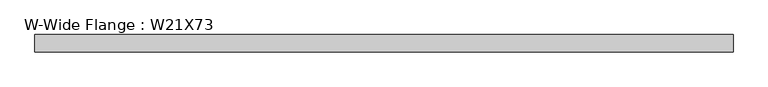
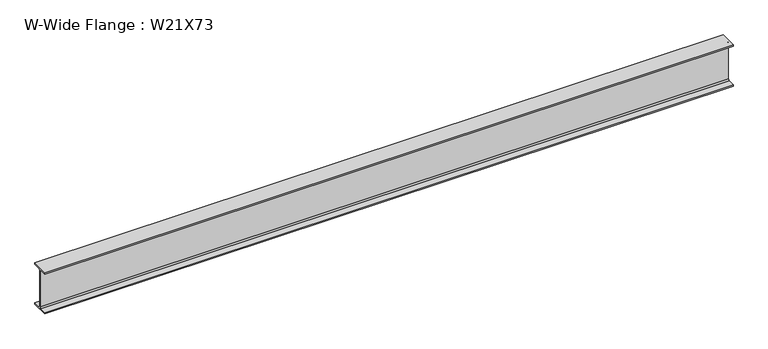
"""IFC4 building model written with IfcOpenShell, lengths in millimetres: beam geometry, W-Wide Flange : W21X73."""

from ifc_helpers import new_model, si_unit, point, frame, frame_2d, origin, place, context, project, spatial, polyline, circle_curve, trimmed, segment, composite_curve, outline, extrude, source, transform, mapped, element, save


def w_wide_flange_w21x73_6fdf119d(model_context):
    return source(origin(), model_context, "Body", "SweptSolid", [
        extrude(outline(composite_curve([segment(polyline([(105.41, -250.444), (105.41, -269.24), (-105.41, -269.24), (-105.41, -250.444), (-23.495, -250.444)]), True, "CONTINUOUS"), segment(trimmed(circle_curve(frame_2d((-23.495, -232.7275)), 17.7165), [point((-23.495, -250.444))], [point((-5.7785, -232.7275))], True, "CARTESIAN"), True, "CONTINUOUS"), segment(polyline([(-5.7785, -232.7275), (-5.7785, 232.7275)]), True, "CONTINUOUS"), segment(trimmed(circle_curve(frame_2d((-23.495, 232.7275)), 17.7165), [point((-5.7785, 232.7275))], [point((-23.495, 250.444))], True, "CARTESIAN"), True, "CONTINUOUS"), segment(polyline([(-23.495, 250.444), (-105.41, 250.444), (-105.41, 269.24), (105.41, 269.24), (105.41, 250.444), (23.495, 250.444)]), True, "CONTINUOUS"), segment(trimmed(circle_curve(frame_2d((23.495, 232.7275)), 17.7165), [point((23.495, 250.444))], [point((5.7785, 232.7275))], True, "CARTESIAN"), True, "CONTINUOUS"), segment(polyline([(5.7785, 232.7275), (5.7785, -232.7275)]), True, "CONTINUOUS"), segment(trimmed(circle_curve(frame_2d((23.495, -232.7275)), 17.7165), [point((5.7785, -232.7275))], [point((23.495, -250.444))], True, "CARTESIAN"), True, "CONTINUOUS"), segment(polyline([(23.495, -250.444), (105.41, -250.444)]), True, "CONTINUOUS")], self_intersect=False)), frame((-4243.07, 0.0, 0.0), z_axis=(1.0, 0.0, 0.0), x_axis=(0.0, 1.0, 0.0)), (0.0, 0.0, 1.0), 8483.6),
    ])


if __name__ == "__main__":
    model = new_model("IFC4")
    model_context = context("Model", 3, world=origin())
    ifc_project = project(units=[si_unit("LENGTHUNIT", "METRE", prefix="MILLI")], contexts=[model_context])
    site = spatial("IfcSite", under=ifc_project)
    building = spatial("IfcBuilding", under=site)
    placement = place(None, origin())
    w_wide_flange_w21x73_shape = w_wide_flange_w21x73_6fdf119d(model_context)
    element("IfcBeam", 1, ObjectType="W-Wide Flange : W21X73", at=placement, inside=building, context=model_context, shape_type="MappedRepresentation", body=[
        mapped(w_wide_flange_w21x73_shape, transform((0.0, 0.0, 0.0), x_axis=(1.0, 0.0, 0.0), y_axis=(0.0, 1.0, 0.0), z_axis=(0.0, 0.0, 1.0))),
    ])
    save(model, "model.ifc")

# Revit data of these elements
# Type "W-Wide Flange : W21X73"
#   Assembly Code = "B10"
#   W = 73
#   Start Extension Calculation [instance default] = 10' - 0"
#   Start Extension [instance default] = -0' - 0 1/2"
#   End Extension Calculation [instance default] = 10' - 0"
#   End Extension [instance default] = -0' - 0 1/2"
#   Length [instance default] = 5' - 0"
#   bf = 0' - 8.3"
#   d = 1' - 9.2"
#   k = 0' - 1 7/16"
#   k2 = 0' - 0.6975"
#   tf = 0' - 0.74"
#   tw = 0' - 0.455"
#   A = 0.149306 SF
#   Beam Material [instance default] = Metal - Steel - ASTM A992
# Element 1 (IfcBeam, "W-Wide Flange : W21X73")
#   Materials on its faces: "Metal - Steel - ASTM A992"
# Materials
#   "Metal - Steel - ASTM A992": class "Metal", colour RGB 128 0 0, transparency 0
